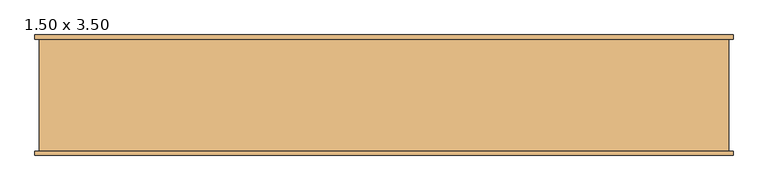
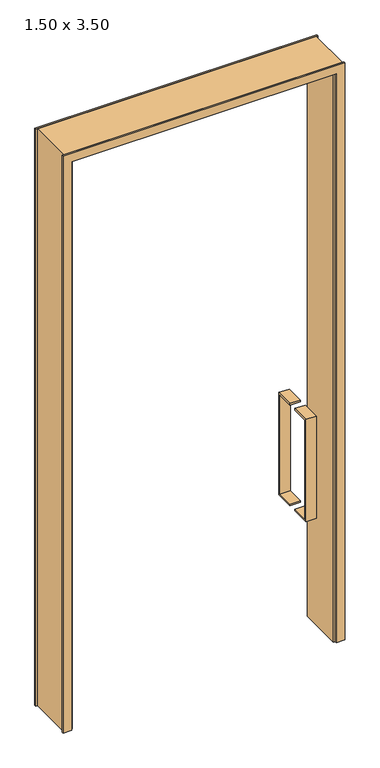
"""IFC4 building model written with IfcOpenShell, lengths in millimetres: door geometry, .CC_ND 300 PORTA PIVOTANTE_COM BANDEIRA_COM EXTENSÃO : 1.50 x 3.50."""

import ifcopenshell
import ifcopenshell.guid

model = None  # the IFC model being written
_history = None  # IfcOwnerHistory: only IFC2X3 demands one
_inside = {}  # id of a spatial element -> (the spatial element, [elements in it])
_under = {}  # id of a project, library or spatial element -> (it, [spatial elements below it])
_declared = {}  # id of a project -> (the project, [libraries it declares])
_typed = {}  # id of a type object -> (the type object, [elements of that type])
_made_of = {}  # id of a material, layer set ... -> (it, [elements and type objects made of it])


def new_model(schema):
    """Start an empty IFC model of exactly this schema.

    Asked for "IFC4X3", IfcOpenShell would pick the latest addendum, in which some entities
    have other attributes; the version numbers below select the first issue.
    IFC2X3 requires an IfcOwnerHistory on every rooted entity: one is made here for all.
    """
    global model, _history
    if schema == "IFC4X3":
        model = ifcopenshell.file(schema_version=(4, 3, 0, 0))
    else:
        model = ifcopenshell.file(schema=schema)
    _inside.clear()
    _under.clear()
    _declared.clear()
    _typed.clear()
    _made_of.clear()
    _history = None
    if model.schema == "IFC2X3":
        org = make("IfcOrganization", Name="unknown")
        user = make(
            "IfcPersonAndOrganization",
            ThePerson=make("IfcPerson", FamilyName="unknown"),
            TheOrganization=org,
        )
        app = make(
            "IfcApplication",
            ApplicationDeveloper=org,
            Version="unknown",
            ApplicationFullName="unknown",
            ApplicationIdentifier="unknown",
        )
        _history = make(
            "IfcOwnerHistory",
            OwningUser=user,
            OwningApplication=app,
            ChangeAction="ADDED",
            CreationDate=0,
        )
    return model


def make(cls, **values):
    """One entity of the class cls with the attributes given. An attribute that is None is left unset."""
    return model.create_entity(
        cls, **{name: value for name, value in values.items() if value is not None}
    )


def rooted(cls, **values):
    """An entity with a GlobalId (a new one), such as an element, a storey or a relation."""
    return make(cls, GlobalId=ifcopenshell.guid.new(), OwnerHistory=_history, **values)


def si_unit(unit_type, name, prefix=None):
    """IfcSIUnit, for example si_unit("LENGTHUNIT", "METRE", prefix="MILLI")."""
    return make("IfcSIUnit", UnitType=unit_type, Prefix=prefix, Name=name)


def assignment(units):
    """IfcUnitAssignment: the units of a project."""
    return None if units is None else make("IfcUnitAssignment", Units=units)


def point(xyz):
    """IfcCartesianPoint."""
    return None if xyz is None else make("IfcCartesianPoint", Coordinates=xyz)


def direction(xyz):
    """IfcDirection."""
    return None if xyz is None else make("IfcDirection", DirectionRatios=xyz)


def frame(location, z_axis=None, x_axis=None):
    """IfcAxis2Placement3D, a coordinate frame: its origin and axes. An axis left out is left unset."""
    return make(
        "IfcAxis2Placement3D",
        Location=point(location),
        Axis=direction(z_axis),
        RefDirection=direction(x_axis),
    )


def origin():
    """The frame at (0, 0, 0) with its axes left unset."""
    return frame((0.0, 0.0, 0.0))


def place(relative_to, where):
    """IfcLocalPlacement: puts the frame where relative to a parent placement (None: the world)."""
    return make(
        "IfcLocalPlacement", PlacementRelTo=relative_to, RelativePlacement=where
    )


def context(
    kind, dimensions, precision=None, world=None, true_north=None, identifier=None
):
    """IfcGeometricRepresentationContext, for example the 3D "Model" context."""
    return make(
        "IfcGeometricRepresentationContext",
        ContextIdentifier=identifier,
        ContextType=kind,
        CoordinateSpaceDimension=dimensions,
        Precision=precision,
        WorldCoordinateSystem=world,
        TrueNorth=true_north,
    )


def project(units=None, contexts=None):
    """IfcProject with its units and contexts."""
    return rooted(
        "IfcProject",
        Name="project",
        RepresentationContexts=contexts,
        UnitsInContext=assignment(units),
    )


def spatial(cls, under=None, at=None, **own):
    """A site, building, storey or space (cls), placed at a placement, below another one or the project."""
    s = rooted(cls, ObjectPlacement=at, **own)
    if under is not None:
        _under.setdefault(under.id(), (under, []))[1].append(s)
    return s


def polyline(points):
    """IfcPolyline through the points."""
    return make("IfcPolyline", Points=[point(p) for p in points])


def outline(outer, holes=None, kind="AREA"):
    """IfcArbitraryClosedProfileDef: a profile drawn as a closed curve; with holes, ...WithVoids."""
    if holes is None:
        return make("IfcArbitraryClosedProfileDef", ProfileType=kind, OuterCurve=outer)
    return make(
        "IfcArbitraryProfileDefWithVoids",
        ProfileType=kind,
        OuterCurve=outer,
        InnerCurves=holes,
    )


def extrude(swept, where, along, depth):
    """IfcExtrudedAreaSolid: the profile swept, set in the frame where, extruded along a direction by depth."""
    return make(
        "IfcExtrudedAreaSolid",
        SweptArea=swept,
        Position=where,
        ExtrudedDirection=direction(along),
        Depth=depth,
    )


def shape(context_of_items, identifier, shape_type, items):
    """IfcShapeRepresentation: the items that make up one representation, for example the "Body"."""
    return make(
        "IfcShapeRepresentation",
        ContextOfItems=context_of_items,
        RepresentationIdentifier=identifier,
        RepresentationType=shape_type,
        Items=items,
    )


def source(mapping_origin, context_of_items, identifier, shape_type, items):
    """IfcRepresentationMap: a shape defined once, which mapped items show again and again."""
    return make(
        "IfcRepresentationMap",
        MappingOrigin=mapping_origin,
        MappedRepresentation=shape(context_of_items, identifier, shape_type, items),
    )


def transform(
    local_origin,
    x_axis=None,
    y_axis=None,
    z_axis=None,
    scale=None,
    scale2=None,
    scale3=None,
    uniform=True,
):
    """IfcCartesianTransformationOperator3D, or its non-uniform kind. x_axis, y_axis, z_axis: its Axis1, 2, 3."""
    if uniform:
        return make(
            "IfcCartesianTransformationOperator3D",
            Axis1=direction(x_axis),
            Axis2=direction(y_axis),
            LocalOrigin=point(local_origin),
            Scale=scale,
            Axis3=direction(z_axis),
        )
    return make(
        "IfcCartesianTransformationOperator3DnonUniform",
        Axis1=direction(x_axis),
        Axis2=direction(y_axis),
        LocalOrigin=point(local_origin),
        Scale=scale,
        Axis3=direction(z_axis),
        Scale2=scale2,
        Scale3=scale3,
    )


def mapped(mapping_source, mapping_target):
    """IfcMappedItem: shows the shape of a source again, moved by a transform."""
    return make(
        "IfcMappedItem", MappingSource=mapping_source, MappingTarget=mapping_target
    )


def made_of(thing, what):
    """Note that an element or type object is made of a material, layer set ...; save() writes the relation."""
    if what is not None:
        _made_of.setdefault(what.id(), (what, []))[1].append(thing)
    return thing


def element(
    cls,
    number,
    at=None,
    inside=None,
    cuts=None,
    type_object=None,
    material=None,
    context=None,
    identifier="Body",
    shape_type=None,
    held_by="IfcProductDefinitionShape",
    body=None,
    shapes=None,
    **own,
):
    """One element of the class cls, such as IfcWall. Its Tag is "e" and its number.

    at: its placement. inside: the storey or other place that contains it. cuts: it is an
    opening in that element (IfcRelVoidsElement). A single representation is given by context,
    identifier, shape_type and body (its items); several are given by shapes. held_by: the class
    of the entity that holds the representations. save() writes the other relations.
    """
    e = rooted(cls, Tag="e%d" % number, ObjectPlacement=at, **own)
    if body is not None:
        shapes = [shape(context, identifier, shape_type, body)]
    if shapes is not None:
        e.Representation = make(held_by, Representations=shapes)
    if inside is not None:
        _inside.setdefault(inside.id(), (inside, []))[1].append(e)
    if cuts is not None:
        rooted(
            "IfcRelVoidsElement", RelatingBuildingElement=cuts, RelatedOpeningElement=e
        )
    if type_object is not None:
        _typed.setdefault(type_object.id(), (type_object, []))[1].append(e)
    return made_of(e, material)


def aggregate(whole, parts):
    """IfcRelAggregates: a whole, such as a stair, and the parts it consists of."""
    return rooted("IfcRelAggregates", RelatingObject=whole, RelatedObjects=parts)


def save(model, path):
    """Write the relations noted so far, then the file.

    IfcRelAggregates (storeys below a building ...), IfcRelContainedInSpatialStructure (elements
    in a storey), IfcRelDefinesByType, IfcRelAssociatesMaterial and IfcRelDeclares: one each for
    every whole, place, type object, material and project.
    """
    for whole, parts in _under.values():
        aggregate(whole, parts)
    for where, things in _inside.values():
        rooted(
            "IfcRelContainedInSpatialStructure",
            RelatedElements=things,
            RelatingStructure=where,
        )
    for kind, things in _typed.values():
        rooted("IfcRelDefinesByType", RelatedObjects=things, RelatingType=kind)
    for what, things in _made_of.values():
        rooted("IfcRelAssociatesMaterial", RelatedObjects=things, RelatingMaterial=what)
    for by, libraries in _declared.values():
        rooted("IfcRelDeclares", RelatingContext=by, RelatedDefinitions=libraries)
    model.write(path)


def door_1_50_x_3_50_a1620f17(model_context):
    return source(origin(), model_context, "Body", "SweptSolid", [
        extrude(outline(polyline([(0.0, -810.0), (0.0, -760.0), (3450.0, -760.0), (3450.0, 760.0), (0.0, 760.0), (0.0, 810.0), (3500.0, 810.0), (3500.0, -810.0), (0.0, -810.0)])), frame((0.0, -139.9, 0.0), z_axis=(0.0, 1.0, 0.0), x_axis=(0.0, 0.0, 1.0)), (0.0, 0.0, 1.0), 10.0),
        extrude(outline(polyline([(0.0, 760.0), (0.0, 810.0), (3500.0, 810.0), (3500.0, -810.0), (0.0, -810.0), (0.0, -760.0), (3450.0, -760.0), (3450.0, 760.0), (0.0, 760.0)])), frame((0.0, 129.9, 0.0), z_axis=(0.0, 1.0, 0.0), x_axis=(0.0, 0.0, 1.0)), (0.0, 0.0, 1.0), 10.0),
        extrude(outline(polyline([(0.0, -800.0), (0.0, -750.0), (3450.0, -750.0), (3450.0, 750.0), (0.0, 750.0), (0.0, 800.0), (3500.0, 800.0), (3500.0, -800.0), (0.0, -800.0)])), frame((0.0, -129.9, 0.0), z_axis=(0.0, 1.0, 0.0), x_axis=(0.0, 0.0, 1.0)), (0.0, 0.0, 1.0), 259.8),
        extrude(outline(polyline([(-25.0, 1410.0), (-25.0, 1400.0), (-125.0, 1400.0), (-125.0, 800.0), (-25.0, 800.0), (-25.0, 790.0), (-135.0, 790.0), (-135.0, 1410.0), (-25.0, 1410.0)])), frame((590.0, 0.0, 0.0), z_axis=(1.0, 0.0, 0.0), x_axis=(0.0, 1.0, 0.0)), (0.0, 0.0, 1.0), 60.0),
        extrude(outline(polyline([(25.0, 1400.0), (25.0, 1410.0), (135.0, 1410.0), (135.0, 790.0), (25.0, 790.0), (25.0, 800.0), (125.0, 800.0), (125.0, 1400.0), (25.0, 1400.0)])), frame((590.0, 0.0, 0.0), z_axis=(1.0, 0.0, 0.0), x_axis=(0.0, 1.0, 0.0)), (0.0, 0.0, 1.0), 60.0),
    ])


if __name__ == "__main__":
    model = new_model("IFC4")
    model_context = context("Model", 3, world=origin())
    ifc_project = project(units=[si_unit("LENGTHUNIT", "METRE", prefix="MILLI")], contexts=[model_context])
    site = spatial("IfcSite", under=ifc_project)
    building = spatial("IfcBuilding", under=site)
    placement = place(None, origin())
    door_1_50_x_3_50_shape = door_1_50_x_3_50_a1620f17(model_context)
    element("IfcDoor", 1, ObjectType=".CC_ND 300 PORTA PIVOTANTE_COM BANDEIRA_COM EXTENSÃO : 1.50 x 3.50", at=placement, inside=building, context=model_context, shape_type="MappedRepresentation", body=[
        mapped(door_1_50_x_3_50_shape, transform((0.0, 0.0, 0.0), x_axis=(1.0, 0.0, 0.0), y_axis=(0.0, 1.0, 0.0), z_axis=(0.0, 0.0, 1.0))),
    ])
    save(model, "model.ifc")

# Revit data of these elements
# Type ".CC_ND 300 PORTA PIVOTANTE_COM BANDEIRA_COM EXTENSÃO : 1.50 x 3.50"
#   Type Mark = "151"
#   Pivot = 0.10 m
#   Largura moldura = 0.05 m
#   Rough Width = 1.60 m
#   Extensão do acabamento interior [instance default] = 0.00 m
#   Extensão do acabamento exterior [instance default] = 0.00 m
#   Espessura moldura = 0.01 m
#   Espessura batente = 0.05 m
#   Thickness = 0.05 m
#   Rough Height = 3.50 m
#   Altura bandeira = 1.35 m
#   Height = 2.10 m
#   Width = 1.50 m
#   Puxador interno [instance default] = yes
#   Puxador externo [instance default] = yes
#   Número de ripas da porta = 4
#   Moldura interna [instance default] = yes
#   Moldura externa [instance default] = yes
#   Function = 1
#   Puxador = .ALUMÍNIO
#   Porta = .MADEIRA_CEREJEIRA CLARO
#   Moldura = .MADEIRA_CEREJEIRA CLARO
#   Batente = .MADEIRA_CEREJEIRA CLARO
#   Wall Closure = (empty or 0)
# Element 1 (IfcDoor, ".CC_ND 300 PORTA PIVOTANTE_COM BANDEIRA_COM EXTENSÃO : 1.50 x 3.50")
#   Materials on its faces: ".MADEIRA_CEREJEIRA CLARO", ".ALUMÍNIO"
# Materials
#   ".ALUMÍNIO": class "CC_METAIS", colour RGB 244 244 244, transparency 0, Description = "Material alumínio", Cost = 0
#   ".MADEIRA_CEREJEIRA CLARO": class ".CC_MADEIRA REVEST.", colour RGB 233 182 144, transparency 0, Cost = 0
